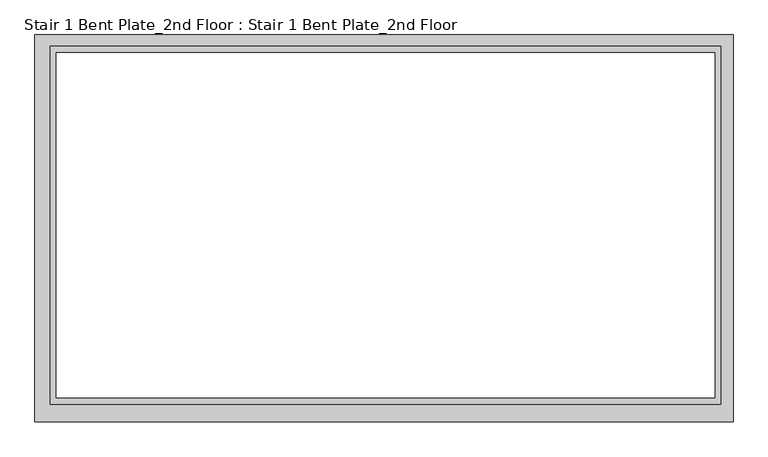
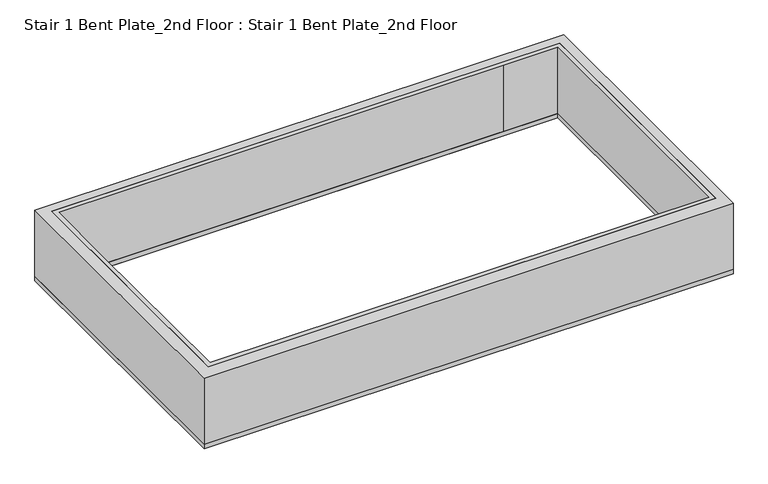
"""IFC4 building model written with IfcOpenShell, lengths in millimetres: proxy geometry, Stair 1 Bent Plate_2nd Floor : Stair 1 Bent Plate_2nd Floor."""

from ifc_helpers import new_model, si_unit, frame, origin, origin_with_axes, place, context, project, spatial, polyline, outline, extrude, source, transform, mapped, element, save


def stair_1_bent_plate_2nd_floor_stair_1_bent_plate_2nd_floor_c3bc87a6(model_context):
    return source(origin(), model_context, "Body", "SweptSolid", [
        extrude(outline(polyline([(-279.4, -750.8875), (-279.4, 46.0375), (1158.875, 46.0375), (1158.875, -750.8875), (-279.4, -750.8875)]), holes=[polyline([(1133.475, 22.225), (-247.65, 22.225), (-247.65, -714.375), (1133.475, -714.375), (1133.475, 22.225)])]), frame((0.0, 0.0, 12.7), z_axis=(0.0, 0.0, 1.0), x_axis=(1.0, 0.0, 0.0)), (0.0, 0.0, 1.0), 190.5),
        extrude(outline(polyline([(1158.875, -750.8875), (-279.4, -750.8875), (-279.4, 46.0375), (1158.875, 46.0375), (1158.875, -750.8875)]), holes=[polyline([(-234.95, 9.525), (-234.95, -701.675), (1120.775, -701.675), (1120.775, 9.525), (-234.95, 9.525)])]), origin_with_axes(), (0.0, 0.0, 1.0), 12.7),
        extrude(outline(polyline([(1133.475, 22.225), (1133.475, -714.375), (-247.65, -714.375), (-247.65, 22.225), (1133.475, 22.225)]), holes=[polyline([(-234.95, -701.675), (1120.775, -701.675), (1120.775, 9.525), (974.725, 9.525), (-234.95, 9.525), (-234.95, -190.5), (-234.95, -701.675)])]), origin_with_axes(), (0.0, 0.0, 1.0), 203.2),
    ])


if __name__ == "__main__":
    model = new_model("IFC4")
    model_context = context("Model", 3, world=origin())
    ifc_project = project(units=[si_unit("LENGTHUNIT", "METRE", prefix="MILLI")], contexts=[model_context])
    site = spatial("IfcSite", under=ifc_project)
    building = spatial("IfcBuilding", under=site)
    placement = place(None, origin())
    stair_1_bent_plate_2nd_floor_stair_1_bent_plate_2nd_floor_shape = stair_1_bent_plate_2nd_floor_stair_1_bent_plate_2nd_floor_c3bc87a6(model_context)
    element("IfcBuildingElementProxy", 1, Name="Stair 1 Bent Plate_2nd Floor : Stair 1 Bent Plate_2nd Floor", ObjectType="Stair 1 Bent Plate_2nd Floor : Stair 1 Bent Plate_2nd Floor", at=placement, inside=building, context=model_context, shape_type="MappedRepresentation", body=[
        mapped(stair_1_bent_plate_2nd_floor_stair_1_bent_plate_2nd_floor_shape, transform((0.0, 0.0, 0.0), x_axis=(1.0, 0.0, 0.0), y_axis=(0.0, 1.0, 0.0), z_axis=(0.0, 0.0, 1.0))),
    ])
    save(model, "model.ifc")

# Revit data of these elements
# Element 1 (IfcBuildingElementProxy, "Stair 1 Bent Plate_2nd Floor : Stair 1 Bent Plate_2nd Floor")
#   Materials on its faces: "Concrete Infill"
# Materials
#   "Concrete Infill": class "Generic", colour RGB 0 255 0, transparency 0, Cost = 0
